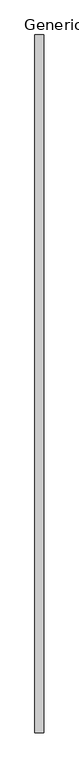
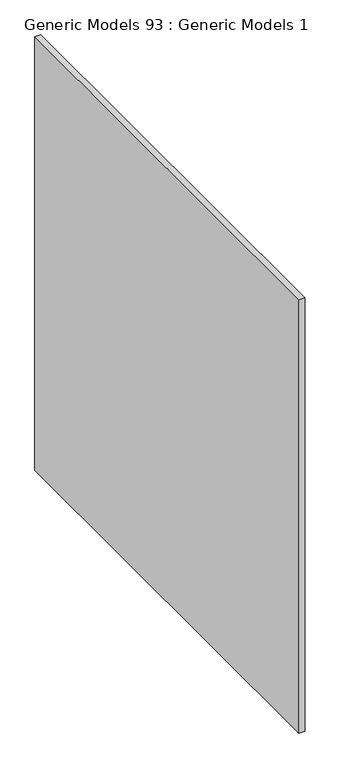
"""IFC4 building model written with IfcOpenShell, lengths in millimetres: proxy geometry, Generic Models 93 : Generic Models 1."""

from ifc_helpers import new_model, si_unit, frame, origin, place, context, project, spatial, polyline, outline, extrude, source, transform, mapped, element, save


def generic_models_93_generic_models_1_66edd626(model_context):
    return source(origin(), model_context, "Body", "SweptSolid", [
        extrude(outline(polyline([(46951.7485531, 1219.2), (46951.7485531, 0.0), (46935.8735531, 0.0), (46935.8735531, 1219.2), (46951.7485531, 1219.2)])), frame((0.0, 0.0, 999.573933), z_axis=(0.0, 0.0, 1.0), x_axis=(1.0, 0.0, 0.0)), (0.0, 0.0, 1.0), 1219.2),
    ])


if __name__ == "__main__":
    model = new_model("IFC4")
    model_context = context("Model", 3, world=origin())
    ifc_project = project(units=[si_unit("LENGTHUNIT", "METRE", prefix="MILLI")], contexts=[model_context])
    site = spatial("IfcSite", under=ifc_project)
    building = spatial("IfcBuilding", under=site)
    placement = place(None, origin())
    generic_models_93_generic_models_1_shape = generic_models_93_generic_models_1_66edd626(model_context)
    element("IfcBuildingElementProxy", 1, Name="Generic Models 93 : Generic Models 1", ObjectType="Generic Models 93 : Generic Models 1", at=placement, inside=building, context=model_context, shape_type="MappedRepresentation", body=[
        mapped(generic_models_93_generic_models_1_shape, transform((0.0, 0.0, 0.0), x_axis=(1.0, 0.0, 0.0), y_axis=(0.0, 1.0, 0.0), z_axis=(0.0, 0.0, 1.0))),
    ])
    save(model, "model.ifc")

# Revit data of these elements
# Element 1 (IfcBuildingElementProxy, "Generic Models 93 : Generic Models 1")
#   Materials on its faces: "5/8\" GYP. BD"
# Materials
#   "5/8\" GYP. BD": class "Generic", colour RGB 255 255 255, transparency 0, Description = "Gypsum Wall Board", Cost = 0
